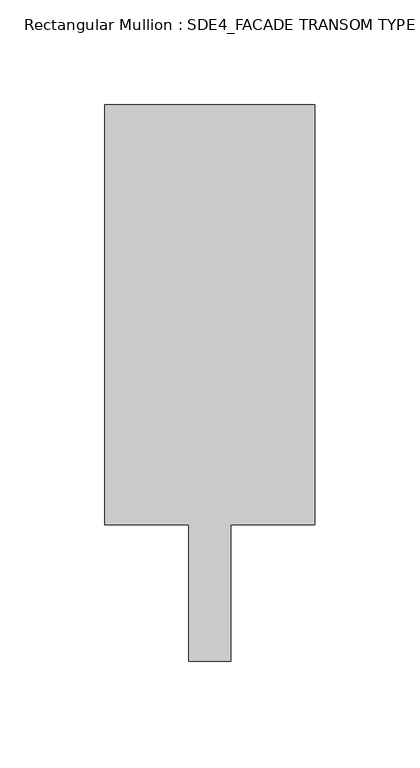
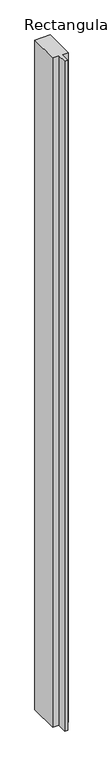
"""IFC4 building model written with IfcOpenShell, lengths in millimetres: member geometry, Rectangular Mullion : SDE4_FACADE TRANSOM TYPE 2."""

from ifc_helpers import new_model, si_unit, frame, origin, place, context, project, spatial, polyline, outline, extrude, source, transform, mapped, element, save


def rectangular_mullion_sde4_facade_transom_type_2_72395da9(model_context):
    return source(origin(), model_context, "Body", "SweptSolid", [
        extrude(outline(polyline([(50.0, 132.5), (50.0, -67.5), (10.0, -67.5), (10.0, -132.5), (-10.0, -132.5), (-10.0, -67.5), (-50.0, -67.5), (-50.0, 132.5), (50.0, 132.5)])), frame((0.0, 0.0, -4578.0), z_axis=(0.0, 0.0, 1.0), x_axis=(1.0, 0.0, 0.0)), (0.0, 0.0, 1.0), 4578.0),
    ])


if __name__ == "__main__":
    model = new_model("IFC4")
    model_context = context("Model", 3, world=origin())
    ifc_project = project(units=[si_unit("LENGTHUNIT", "METRE", prefix="MILLI")], contexts=[model_context])
    site = spatial("IfcSite", under=ifc_project)
    building = spatial("IfcBuilding", under=site)
    placement = place(None, origin())
    rectangular_mullion_sde4_facade_transom_type_2_shape = rectangular_mullion_sde4_facade_transom_type_2_72395da9(model_context)
    element("IfcMember", 1, ObjectType="Rectangular Mullion : SDE4_FACADE TRANSOM TYPE 2", at=placement, inside=building, context=model_context, shape_type="MappedRepresentation", body=[
        mapped(rectangular_mullion_sde4_facade_transom_type_2_shape, transform((0.0, 0.0, 0.0), x_axis=(1.0, 0.0, 0.0), y_axis=(0.0, 1.0, 0.0), z_axis=(0.0, 0.0, 1.0))),
    ])
    save(model, "model.ifc")

# Revit data of these elements
# Type "Rectangular Mullion : SDE4_FACADE TRANSOM TYPE 2"
#   built-in parameter 1007322 = 0.869423 (stored number, unit not read)
#   built-in parameter 1007321 = 0.164042 (stored number, unit not read)
#   built-in parameter 1007320 = 0.164042 (stored number, unit not read)
